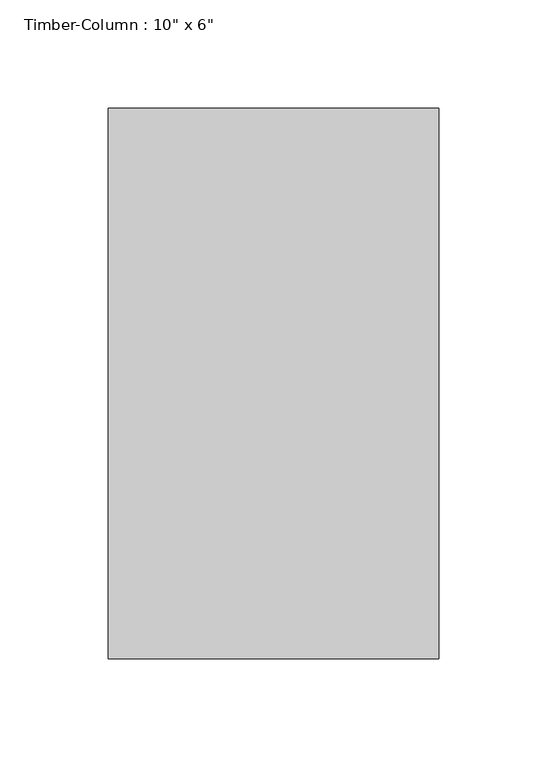
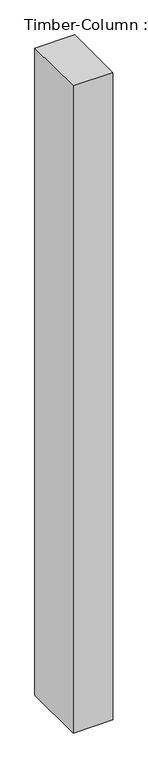
"""IFC4 building model written with IfcOpenShell, lengths in millimetres: column geometry."""

from ifc_helpers import new_model, si_unit, origin, origin_with_axes, place, context, project, spatial, polyline, outline, extrude, source, transform, mapped, element, save


def column_1c9a027e(model_context):
    return source(origin(), model_context, "Body", "SweptSolid", [
        extrude(outline(polyline([(76.2, 127.0), (76.2, -127.0), (-76.2, -127.0), (-76.2, 127.0), (76.2, 127.0)])), origin_with_axes(), (0.0, 0.0, 1.0), 2628.9),
    ])


if __name__ == "__main__":
    model = new_model("IFC4")
    model_context = context("Model", 3, world=origin())
    ifc_project = project(units=[si_unit("LENGTHUNIT", "METRE", prefix="MILLI")], contexts=[model_context])
    site = spatial("IfcSite", under=ifc_project)
    building = spatial("IfcBuilding", under=site)
    placement = place(None, origin())
    column_shape = column_1c9a027e(model_context)
    element("IfcColumn", 1, ObjectType="Timber-Column : 10\" x 6\"", at=placement, inside=building, context=model_context, shape_type="MappedRepresentation", body=[
        mapped(column_shape, transform((0.0, 0.0, 0.0), x_axis=(1.0, 0.0, 0.0), y_axis=(0.0, 1.0, 0.0), z_axis=(0.0, 0.0, 1.0))),
    ])
    save(model, "model.ifc")

# Revit data of these elements
# Type "Timber-Column : 10\" x 6\""
#   Assembly Code = "B10"
#   A = 0.140625 SF
#   b = 0' - 6"
#   d = 0' - 10"
#   Structural Material [instance default] = Softwood, Lumber
# Element 1 (IfcColumn, "Timber-Column : 10\" x 6\"")
#   Materials on its faces: "Softwood, Lumber"
# Materials
#   "Softwood, Lumber": class "Wood", colour RGB 144 113 62, transparency 0, Description = "Pinus Echinata", Cost = 0
